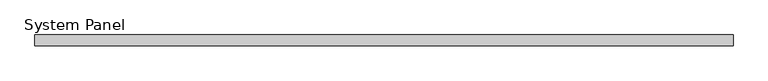
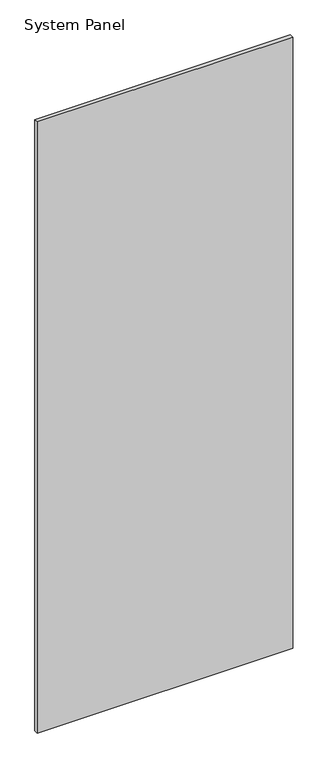
"""IFC4 building model written with IfcOpenShell, lengths in millimetres: plate geometry, System Panel : WWm-Glass-20mm-10mmOffset."""

from ifc_helpers import new_model, si_unit, origin, origin_with_axes, place, context, project, spatial, polyline, outline, extrude, source, transform, mapped, element, save


def system_panel_aade4185(model_context):
    return source(origin(), model_context, "Body", "SweptSolid", [
        extrude(outline(polyline([(642.6694302, 0.0), (-642.6694302, 0.0), (-642.6694302, 20.0), (642.6694302, 20.0), (642.6694302, 0.0)])), origin_with_axes(), (0.0, 0.0, 1.0), 3250.0),
    ])


if __name__ == "__main__":
    model = new_model("IFC4")
    model_context = context("Model", 3, world=origin())
    ifc_project = project(units=[si_unit("LENGTHUNIT", "METRE", prefix="MILLI")], contexts=[model_context])
    site = spatial("IfcSite", under=ifc_project)
    building = spatial("IfcBuilding", under=site)
    placement = place(None, origin())
    system_panel_shape = system_panel_aade4185(model_context)
    element("IfcPlate", 1, ObjectType="System Panel : WWm-Glass-20mm-10mmOffset", at=placement, inside=building, context=model_context, shape_type="MappedRepresentation", body=[
        mapped(system_panel_shape, transform((0.0, 0.0, 0.0), x_axis=(1.0, 0.0, 0.0), y_axis=(0.0, 1.0, 0.0), z_axis=(0.0, 0.0, 1.0))),
    ])
    save(model, "model.ifc")

# Revit data of these elements
# Type "System Panel : WWm-Glass-20mm-10mmOffset"
#   Finish = ""
# Element 1 (IfcPlate, "System Panel : WWm-Glass-20mm-10mmOffset")
#   Materials on its faces: "WW-EC-GL-Storefront"
# Materials
#   "WW-EC-GL-Storefront": class "Glass", colour RGB 236 240 239, transparency 0.85, Description = "Storefront Glass", Cost = 0
